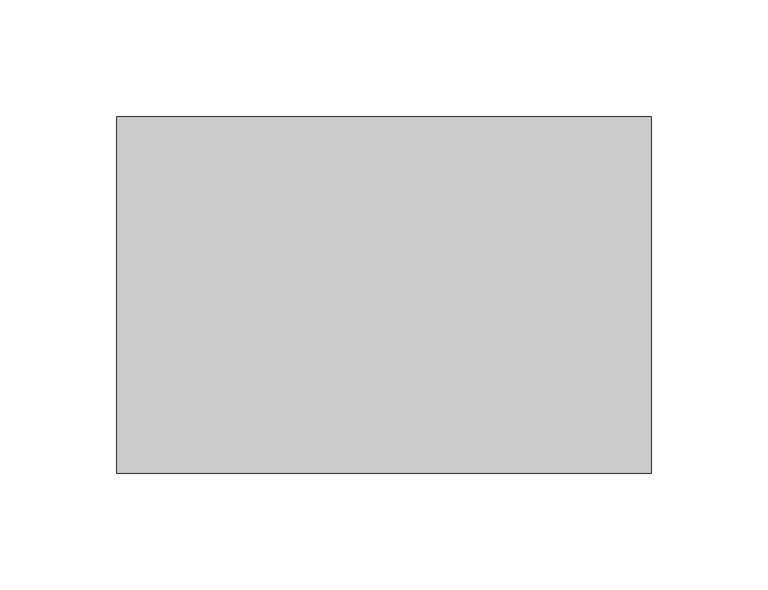
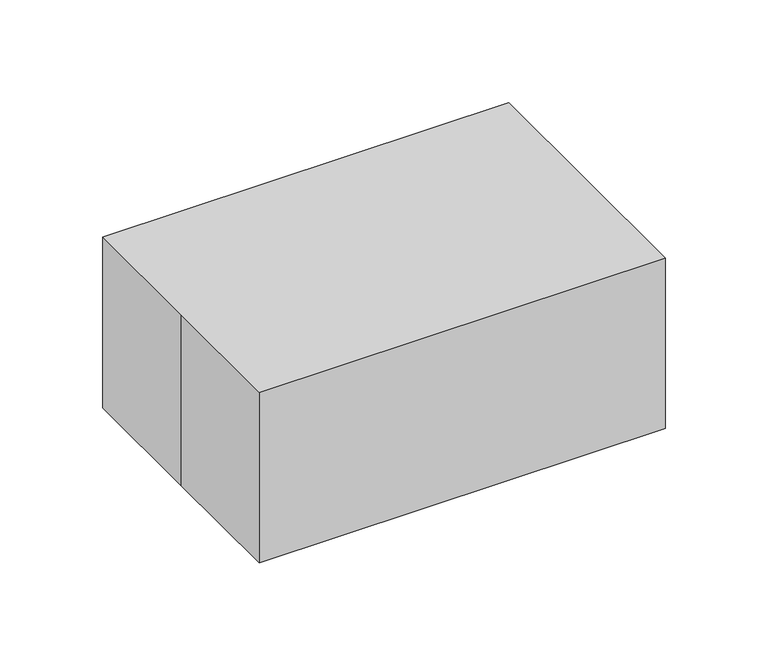
"""IFC4 building model written with IfcOpenShell, lengths in millimetres: proxy geometry, D4260 - Handpiece, Laboratory, Dental, Electric : D4260 - Handpiece, Laboratory, Dental, Electric."""

import ifcopenshell
import ifcopenshell.guid

model = None  # the IFC model being written
_history = None  # IfcOwnerHistory: only IFC2X3 demands one
_inside = {}  # id of a spatial element -> (the spatial element, [elements in it])
_under = {}  # id of a project, library or spatial element -> (it, [spatial elements below it])
_declared = {}  # id of a project -> (the project, [libraries it declares])
_typed = {}  # id of a type object -> (the type object, [elements of that type])
_made_of = {}  # id of a material, layer set ... -> (it, [elements and type objects made of it])


def new_model(schema):
    """Start an empty IFC model of exactly this schema.

    Asked for "IFC4X3", IfcOpenShell would pick the latest addendum, in which some entities
    have other attributes; the version numbers below select the first issue.
    IFC2X3 requires an IfcOwnerHistory on every rooted entity: one is made here for all.
    """
    global model, _history
    if schema == "IFC4X3":
        model = ifcopenshell.file(schema_version=(4, 3, 0, 0))
    else:
        model = ifcopenshell.file(schema=schema)
    _inside.clear()
    _under.clear()
    _declared.clear()
    _typed.clear()
    _made_of.clear()
    _history = None
    if model.schema == "IFC2X3":
        org = make("IfcOrganization", Name="unknown")
        user = make(
            "IfcPersonAndOrganization",
            ThePerson=make("IfcPerson", FamilyName="unknown"),
            TheOrganization=org,
        )
        app = make(
            "IfcApplication",
            ApplicationDeveloper=org,
            Version="unknown",
            ApplicationFullName="unknown",
            ApplicationIdentifier="unknown",
        )
        _history = make(
            "IfcOwnerHistory",
            OwningUser=user,
            OwningApplication=app,
            ChangeAction="ADDED",
            CreationDate=0,
        )
    return model


def make(cls, **values):
    """One entity of the class cls with the attributes given. An attribute that is None is left unset."""
    return model.create_entity(
        cls, **{name: value for name, value in values.items() if value is not None}
    )


def rooted(cls, **values):
    """An entity with a GlobalId (a new one), such as an element, a storey or a relation."""
    return make(cls, GlobalId=ifcopenshell.guid.new(), OwnerHistory=_history, **values)


def si_unit(unit_type, name, prefix=None):
    """IfcSIUnit, for example si_unit("LENGTHUNIT", "METRE", prefix="MILLI")."""
    return make("IfcSIUnit", UnitType=unit_type, Prefix=prefix, Name=name)


def assignment(units):
    """IfcUnitAssignment: the units of a project."""
    return None if units is None else make("IfcUnitAssignment", Units=units)


def point(xyz):
    """IfcCartesianPoint."""
    return None if xyz is None else make("IfcCartesianPoint", Coordinates=xyz)


def direction(xyz):
    """IfcDirection."""
    return None if xyz is None else make("IfcDirection", DirectionRatios=xyz)


def frame(location, z_axis=None, x_axis=None):
    """IfcAxis2Placement3D, a coordinate frame: its origin and axes. An axis left out is left unset."""
    return make(
        "IfcAxis2Placement3D",
        Location=point(location),
        Axis=direction(z_axis),
        RefDirection=direction(x_axis),
    )


def origin():
    """The frame at (0, 0, 0) with its axes left unset."""
    return frame((0.0, 0.0, 0.0))


def origin_with_axes():
    """The frame at (0, 0, 0) with the z axis (0, 0, 1) and the x axis (1, 0, 0) written out."""
    return frame((0.0, 0.0, 0.0), z_axis=(0.0, 0.0, 1.0), x_axis=(1.0, 0.0, 0.0))


def place(relative_to, where):
    """IfcLocalPlacement: puts the frame where relative to a parent placement (None: the world)."""
    return make(
        "IfcLocalPlacement", PlacementRelTo=relative_to, RelativePlacement=where
    )


def context(
    kind, dimensions, precision=None, world=None, true_north=None, identifier=None
):
    """IfcGeometricRepresentationContext, for example the 3D "Model" context."""
    return make(
        "IfcGeometricRepresentationContext",
        ContextIdentifier=identifier,
        ContextType=kind,
        CoordinateSpaceDimension=dimensions,
        Precision=precision,
        WorldCoordinateSystem=world,
        TrueNorth=true_north,
    )


def project(units=None, contexts=None):
    """IfcProject with its units and contexts."""
    return rooted(
        "IfcProject",
        Name="project",
        RepresentationContexts=contexts,
        UnitsInContext=assignment(units),
    )


def spatial(cls, under=None, at=None, **own):
    """A site, building, storey or space (cls), placed at a placement, below another one or the project."""
    s = rooted(cls, ObjectPlacement=at, **own)
    if under is not None:
        _under.setdefault(under.id(), (under, []))[1].append(s)
    return s


def polyline(points):
    """IfcPolyline through the points."""
    return make("IfcPolyline", Points=[point(p) for p in points])


def outline(outer, holes=None, kind="AREA"):
    """IfcArbitraryClosedProfileDef: a profile drawn as a closed curve; with holes, ...WithVoids."""
    if holes is None:
        return make("IfcArbitraryClosedProfileDef", ProfileType=kind, OuterCurve=outer)
    return make(
        "IfcArbitraryProfileDefWithVoids",
        ProfileType=kind,
        OuterCurve=outer,
        InnerCurves=holes,
    )


def extrude(swept, where, along, depth):
    """IfcExtrudedAreaSolid: the profile swept, set in the frame where, extruded along a direction by depth."""
    return make(
        "IfcExtrudedAreaSolid",
        SweptArea=swept,
        Position=where,
        ExtrudedDirection=direction(along),
        Depth=depth,
    )


def shape(context_of_items, identifier, shape_type, items):
    """IfcShapeRepresentation: the items that make up one representation, for example the "Body"."""
    return make(
        "IfcShapeRepresentation",
        ContextOfItems=context_of_items,
        RepresentationIdentifier=identifier,
        RepresentationType=shape_type,
        Items=items,
    )


def source(mapping_origin, context_of_items, identifier, shape_type, items):
    """IfcRepresentationMap: a shape defined once, which mapped items show again and again."""
    return make(
        "IfcRepresentationMap",
        MappingOrigin=mapping_origin,
        MappedRepresentation=shape(context_of_items, identifier, shape_type, items),
    )


def transform(
    local_origin,
    x_axis=None,
    y_axis=None,
    z_axis=None,
    scale=None,
    scale2=None,
    scale3=None,
    uniform=True,
):
    """IfcCartesianTransformationOperator3D, or its non-uniform kind. x_axis, y_axis, z_axis: its Axis1, 2, 3."""
    if uniform:
        return make(
            "IfcCartesianTransformationOperator3D",
            Axis1=direction(x_axis),
            Axis2=direction(y_axis),
            LocalOrigin=point(local_origin),
            Scale=scale,
            Axis3=direction(z_axis),
        )
    return make(
        "IfcCartesianTransformationOperator3DnonUniform",
        Axis1=direction(x_axis),
        Axis2=direction(y_axis),
        LocalOrigin=point(local_origin),
        Scale=scale,
        Axis3=direction(z_axis),
        Scale2=scale2,
        Scale3=scale3,
    )


def mapped(mapping_source, mapping_target):
    """IfcMappedItem: shows the shape of a source again, moved by a transform."""
    return make(
        "IfcMappedItem", MappingSource=mapping_source, MappingTarget=mapping_target
    )


def made_of(thing, what):
    """Note that an element or type object is made of a material, layer set ...; save() writes the relation."""
    if what is not None:
        _made_of.setdefault(what.id(), (what, []))[1].append(thing)
    return thing


def element(
    cls,
    number,
    at=None,
    inside=None,
    cuts=None,
    type_object=None,
    material=None,
    context=None,
    identifier="Body",
    shape_type=None,
    held_by="IfcProductDefinitionShape",
    body=None,
    shapes=None,
    **own,
):
    """One element of the class cls, such as IfcWall. Its Tag is "e" and its number.

    at: its placement. inside: the storey or other place that contains it. cuts: it is an
    opening in that element (IfcRelVoidsElement). A single representation is given by context,
    identifier, shape_type and body (its items); several are given by shapes. held_by: the class
    of the entity that holds the representations. save() writes the other relations.
    """
    e = rooted(cls, Tag="e%d" % number, ObjectPlacement=at, **own)
    if body is not None:
        shapes = [shape(context, identifier, shape_type, body)]
    if shapes is not None:
        e.Representation = make(held_by, Representations=shapes)
    if inside is not None:
        _inside.setdefault(inside.id(), (inside, []))[1].append(e)
    if cuts is not None:
        rooted(
            "IfcRelVoidsElement", RelatingBuildingElement=cuts, RelatedOpeningElement=e
        )
    if type_object is not None:
        _typed.setdefault(type_object.id(), (type_object, []))[1].append(e)
    return made_of(e, material)


def aggregate(whole, parts):
    """IfcRelAggregates: a whole, such as a stair, and the parts it consists of."""
    return rooted("IfcRelAggregates", RelatingObject=whole, RelatedObjects=parts)


def save(model, path):
    """Write the relations noted so far, then the file.

    IfcRelAggregates (storeys below a building ...), IfcRelContainedInSpatialStructure (elements
    in a storey), IfcRelDefinesByType, IfcRelAssociatesMaterial and IfcRelDeclares: one each for
    every whole, place, type object, material and project.
    """
    for whole, parts in _under.values():
        aggregate(whole, parts)
    for where, things in _inside.values():
        rooted(
            "IfcRelContainedInSpatialStructure",
            RelatedElements=things,
            RelatingStructure=where,
        )
    for kind, things in _typed.values():
        rooted("IfcRelDefinesByType", RelatedObjects=things, RelatingType=kind)
    for what, things in _made_of.values():
        rooted("IfcRelAssociatesMaterial", RelatedObjects=things, RelatingMaterial=what)
    for by, libraries in _declared.values():
        rooted("IfcRelDeclares", RelatingContext=by, RelatedDefinitions=libraries)
    model.write(path)


def specialty_equipment_62e1c088(model_context):
    return source(origin(), model_context, "Body", "SweptSolid", [
        extrude(outline(polyline([(100.6709579, 63.4814676), (100.6709579, -63.5185324), (-102.5290421, -63.5185324), (-102.5290421, 63.4814676), (100.6709579, 63.4814676)])), origin_with_axes(), (0.0, 0.0, 1.0), 88.9),
        extrude(outline(polyline([(-114.3, 76.2), (114.3, 76.2), (114.3, -76.2), (-114.3, -76.2), (-114.3, 0.0), (-114.3, 76.2)])), origin_with_axes(), (0.0, 0.0, 1.0), 101.6),
    ])


if __name__ == "__main__":
    model = new_model("IFC4")
    model_context = context("Model", 3, world=origin())
    ifc_project = project(units=[si_unit("LENGTHUNIT", "METRE", prefix="MILLI")], contexts=[model_context])
    site = spatial("IfcSite", under=ifc_project)
    building = spatial("IfcBuilding", under=site)
    placement = place(None, origin())
    specialty_equipment_shape = specialty_equipment_62e1c088(model_context)
    element("IfcBuildingElementProxy", 1, Name="D4260 - Handpiece, Laboratory, Dental, Electric : D4260 - Handpiece, Laboratory, Dental, Electric", ObjectType="D4260 - Handpiece, Laboratory, Dental, Electric : D4260 - Handpiece, Laboratory, Dental, Electric", at=placement, inside=building, context=model_context, shape_type="MappedRepresentation", body=[
        mapped(specialty_equipment_shape, transform((0.0, 0.0, 0.0), x_axis=(1.0, 0.0, 0.0), y_axis=(0.0, 1.0, 0.0), z_axis=(0.0, 0.0, 1.0))),
    ])
    save(model, "model.ifc")

# Revit data of these elements
# Project information
#   Room Abbreviation = "DNPL3"
#   Room Description = "Dental Laboratory, Prosthodontic, Full Service (DNPL3)"
#   Sheets - Total = "6"
#   Project Issue Date = "Issue Date"
#   Project Status = "Project Status"
#   Client Name = "Owner"
#   Project Address = "Enter address here"
#   Project Name = "Project Name"
#   Project Number = "Project Number"
#   Publication Date = "1-Feb-16"
# Type "D4260 - Handpiece, Laboratory, Dental, Electric : D4260 - Handpiece, Laboratory, Dental, Electric"
#   Watts2 = "0"
#   Watts1 = "240"
#   Unit_Issue = "EA"
#   UTIL_6_Misc = "-"
#   UTIL_5_NonMedGas = "-"
#   UTIL_4_MiscGas = "-"
#   UTIL_3_MedGas = "-"
#   UTIL_2_Elec = "A"
#   UTIL_1_WaterDrain = "-"
#   Nomenclature = "Handpiece, Laboratory, Dental, Electric"
#   NSN = "6520"
#   Location [instance default] = ""
#   JSN = "D4260"
#   Fund_Source_VA = "-"
#   Fund_Source_Navy = "-"
#   Fund_Source_Army = "-"
#   Fund_Source_AF = "-"
#   ELEC_Volts2 = "0"
#   ELEC_Volts1 = "120"
#   ELEC_Phase2 = "0"
#   ELEC_Phase1 = "1"
#   ELEC_HertzSwitch = "0"
#   ELEC_HertzDependent = "-1"
#   ELEC_Hertz = "60"
#   ELEC_Amps2 = "0"
#   ELEC_Amps1 = "2"
#   DetailDescription = "Portable dental laboratory handpiece. The unit has a straight handle and is electrically powered. The handpiece includes a controller and power cables. Unit is used to grind, polish or finish precious and non-precious metal alloys."
#   CAT_VA = "C"
#   CAT_Navy = "C"
#   CAT_IHS = "-"
#   CAT_Army = "C"
#   CAT_AF = "C"
#   BTUperhour = "0"
#   Weight_IP = 6
#   DIM_Width_IP = 0' - 9"
#   DIM_Height_IP = 0' - 4"
#   DIM_Depth_IP = 0' - 6"
# Element 1 (IfcBuildingElementProxy, "D4260 - Handpiece, Laboratory, Dental, Electric : D4260 - Handpiece, Laboratory, Dental, Electric")
#   Materials on its faces: "EquipSpace"
# Materials
#   "EquipSpace": class "Unassigned", colour RGB 221 217 195, transparency 0.5
